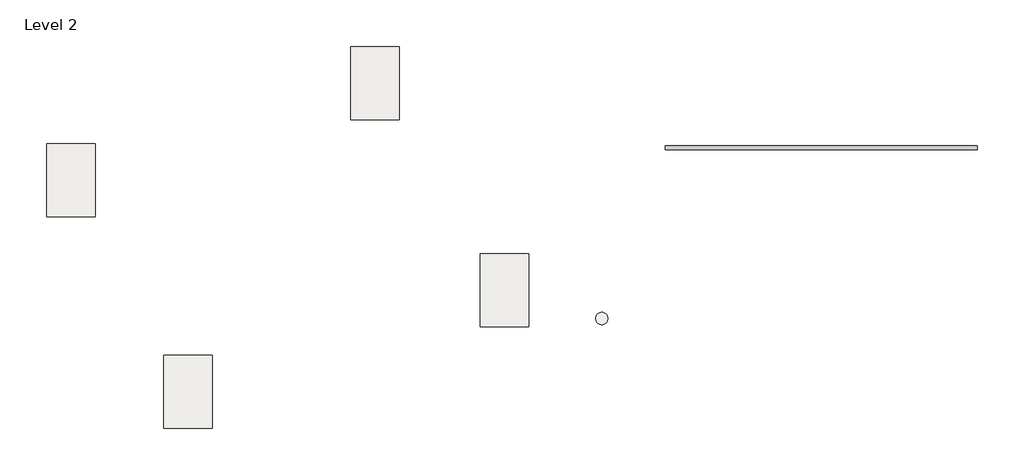
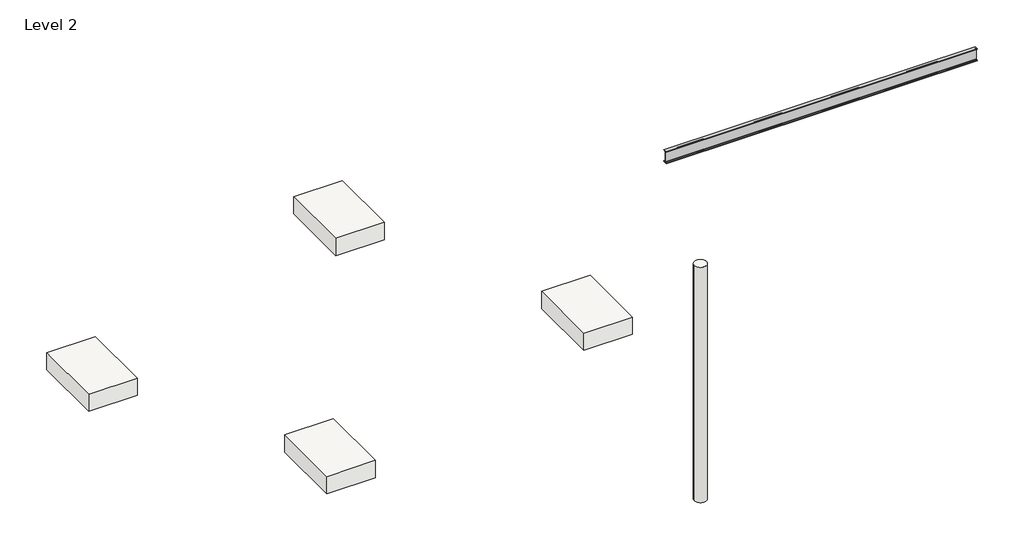
# One storey: 5 slabs, 1 beam.
"""IFC4 building model written with IfcOpenShell, lengths in millimetres."""

import ifcopenshell
import ifcopenshell.guid

model = None  # the IFC model being written
_history = None  # IfcOwnerHistory: only IFC2X3 demands one
_inside = {}  # id of a spatial element -> (the spatial element, [elements in it])
_under = {}  # id of a project, library or spatial element -> (it, [spatial elements below it])
_declared = {}  # id of a project -> (the project, [libraries it declares])
_typed = {}  # id of a type object -> (the type object, [elements of that type])
_made_of = {}  # id of a material, layer set ... -> (it, [elements and type objects made of it])


def new_model(schema):
    """Start an empty IFC model of exactly this schema.

    Asked for "IFC4X3", IfcOpenShell would pick the latest addendum, in which some entities
    have other attributes; the version numbers below select the first issue.
    IFC2X3 requires an IfcOwnerHistory on every rooted entity: one is made here for all.
    """
    global model, _history
    if schema == "IFC4X3":
        model = ifcopenshell.file(schema_version=(4, 3, 0, 0))
    else:
        model = ifcopenshell.file(schema=schema)
    _inside.clear()
    _under.clear()
    _declared.clear()
    _typed.clear()
    _made_of.clear()
    _history = None
    if model.schema == "IFC2X3":
        org = make("IfcOrganization", Name="unknown")
        user = make(
            "IfcPersonAndOrganization",
            ThePerson=make("IfcPerson", FamilyName="unknown"),
            TheOrganization=org,
        )
        app = make(
            "IfcApplication",
            ApplicationDeveloper=org,
            Version="unknown",
            ApplicationFullName="unknown",
            ApplicationIdentifier="unknown",
        )
        _history = make(
            "IfcOwnerHistory",
            OwningUser=user,
            OwningApplication=app,
            ChangeAction="ADDED",
            CreationDate=0,
        )
    return model


def make(cls, **values):
    """One entity of the class cls with the attributes given. An attribute that is None is left unset."""
    return model.create_entity(
        cls, **{name: value for name, value in values.items() if value is not None}
    )


def rooted(cls, **values):
    """An entity with a GlobalId (a new one), such as an element, a storey or a relation."""
    return make(cls, GlobalId=ifcopenshell.guid.new(), OwnerHistory=_history, **values)


def si_unit(unit_type, name, prefix=None):
    """IfcSIUnit, for example si_unit("LENGTHUNIT", "METRE", prefix="MILLI")."""
    return make("IfcSIUnit", UnitType=unit_type, Prefix=prefix, Name=name)


def assignment(units):
    """IfcUnitAssignment: the units of a project."""
    return None if units is None else make("IfcUnitAssignment", Units=units)


def point(xyz):
    """IfcCartesianPoint."""
    return None if xyz is None else make("IfcCartesianPoint", Coordinates=xyz)


def direction(xyz):
    """IfcDirection."""
    return None if xyz is None else make("IfcDirection", DirectionRatios=xyz)


def frame(location, z_axis=None, x_axis=None):
    """IfcAxis2Placement3D, a coordinate frame: its origin and axes. An axis left out is left unset."""
    return make(
        "IfcAxis2Placement3D",
        Location=point(location),
        Axis=direction(z_axis),
        RefDirection=direction(x_axis),
    )


def frame_2d(location, x_axis=None):
    """IfcAxis2Placement2D, a coordinate frame in the plane: its origin and x axis."""
    return make(
        "IfcAxis2Placement2D", Location=point(location), RefDirection=direction(x_axis)
    )


def origin():
    """The frame at (0, 0, 0) with its axes left unset."""
    return frame((0.0, 0.0, 0.0))


def origin_2d():
    """The frame at (0, 0) in the plane with its x axis left unset."""
    return frame_2d((0.0, 0.0))


def place(relative_to, where):
    """IfcLocalPlacement: puts the frame where relative to a parent placement (None: the world)."""
    return make(
        "IfcLocalPlacement", PlacementRelTo=relative_to, RelativePlacement=where
    )


def context(
    kind, dimensions, precision=None, world=None, true_north=None, identifier=None
):
    """IfcGeometricRepresentationContext, for example the 3D "Model" context."""
    return make(
        "IfcGeometricRepresentationContext",
        ContextIdentifier=identifier,
        ContextType=kind,
        CoordinateSpaceDimension=dimensions,
        Precision=precision,
        WorldCoordinateSystem=world,
        TrueNorth=true_north,
    )


def project(units=None, contexts=None):
    """IfcProject with its units and contexts."""
    return rooted(
        "IfcProject",
        Name="project",
        RepresentationContexts=contexts,
        UnitsInContext=assignment(units),
    )


def spatial(cls, under=None, at=None, **own):
    """A site, building, storey or space (cls), placed at a placement, below another one or the project."""
    s = rooted(cls, ObjectPlacement=at, **own)
    if under is not None:
        _under.setdefault(under.id(), (under, []))[1].append(s)
    return s


def polyline(points):
    """IfcPolyline through the points."""
    return make("IfcPolyline", Points=[point(p) for p in points])


def circle_curve(where, radius):
    """IfcCircle in the frame where."""
    return make("IfcCircle", Position=where, Radius=radius)


def trimmed(basis, trim1, trim2, sense, master):
    """IfcTrimmedCurve: the piece of a basis curve between two trims."""
    return make(
        "IfcTrimmedCurve",
        BasisCurve=basis,
        Trim1=trim1,
        Trim2=trim2,
        SenseAgreement=sense,
        MasterRepresentation=master,
    )


def segment(curve, same_sense, transition):
    """IfcCompositeCurveSegment."""
    return make(
        "IfcCompositeCurveSegment",
        Transition=transition,
        SameSense=same_sense,
        ParentCurve=curve,
    )


def composite_curve(segments, self_intersect=None):
    """IfcCompositeCurve: segments joined end to end."""
    return make("IfcCompositeCurve", Segments=segments, SelfIntersect=self_intersect)


def outline(outer, holes=None, kind="AREA"):
    """IfcArbitraryClosedProfileDef: a profile drawn as a closed curve; with holes, ...WithVoids."""
    if holes is None:
        return make("IfcArbitraryClosedProfileDef", ProfileType=kind, OuterCurve=outer)
    return make(
        "IfcArbitraryProfileDefWithVoids",
        ProfileType=kind,
        OuterCurve=outer,
        InnerCurves=holes,
    )


def extrude(swept, where, along, depth):
    """IfcExtrudedAreaSolid: the profile swept, set in the frame where, extruded along a direction by depth."""
    return make(
        "IfcExtrudedAreaSolid",
        SweptArea=swept,
        Position=where,
        ExtrudedDirection=direction(along),
        Depth=depth,
    )


def shape(context_of_items, identifier, shape_type, items):
    """IfcShapeRepresentation: the items that make up one representation, for example the "Body"."""
    return make(
        "IfcShapeRepresentation",
        ContextOfItems=context_of_items,
        RepresentationIdentifier=identifier,
        RepresentationType=shape_type,
        Items=items,
    )


def source(mapping_origin, context_of_items, identifier, shape_type, items):
    """IfcRepresentationMap: a shape defined once, which mapped items show again and again."""
    return make(
        "IfcRepresentationMap",
        MappingOrigin=mapping_origin,
        MappedRepresentation=shape(context_of_items, identifier, shape_type, items),
    )


def transform(
    local_origin,
    x_axis=None,
    y_axis=None,
    z_axis=None,
    scale=None,
    scale2=None,
    scale3=None,
    uniform=True,
):
    """IfcCartesianTransformationOperator3D, or its non-uniform kind. x_axis, y_axis, z_axis: its Axis1, 2, 3."""
    if uniform:
        return make(
            "IfcCartesianTransformationOperator3D",
            Axis1=direction(x_axis),
            Axis2=direction(y_axis),
            LocalOrigin=point(local_origin),
            Scale=scale,
            Axis3=direction(z_axis),
        )
    return make(
        "IfcCartesianTransformationOperator3DnonUniform",
        Axis1=direction(x_axis),
        Axis2=direction(y_axis),
        LocalOrigin=point(local_origin),
        Scale=scale,
        Axis3=direction(z_axis),
        Scale2=scale2,
        Scale3=scale3,
    )


def mapped(mapping_source, mapping_target):
    """IfcMappedItem: shows the shape of a source again, moved by a transform."""
    return make(
        "IfcMappedItem", MappingSource=mapping_source, MappingTarget=mapping_target
    )


def made_of(thing, what):
    """Note that an element or type object is made of a material, layer set ...; save() writes the relation."""
    if what is not None:
        _made_of.setdefault(what.id(), (what, []))[1].append(thing)
    return thing


def element(
    cls,
    number,
    at=None,
    inside=None,
    cuts=None,
    type_object=None,
    material=None,
    context=None,
    identifier="Body",
    shape_type=None,
    held_by="IfcProductDefinitionShape",
    body=None,
    shapes=None,
    **own,
):
    """One element of the class cls, such as IfcWall. Its Tag is "e" and its number.

    at: its placement. inside: the storey or other place that contains it. cuts: it is an
    opening in that element (IfcRelVoidsElement). A single representation is given by context,
    identifier, shape_type and body (its items); several are given by shapes. held_by: the class
    of the entity that holds the representations. save() writes the other relations.
    """
    e = rooted(cls, Tag="e%d" % number, ObjectPlacement=at, **own)
    if body is not None:
        shapes = [shape(context, identifier, shape_type, body)]
    if shapes is not None:
        e.Representation = make(held_by, Representations=shapes)
    if inside is not None:
        _inside.setdefault(inside.id(), (inside, []))[1].append(e)
    if cuts is not None:
        rooted(
            "IfcRelVoidsElement", RelatingBuildingElement=cuts, RelatedOpeningElement=e
        )
    if type_object is not None:
        _typed.setdefault(type_object.id(), (type_object, []))[1].append(e)
    return made_of(e, material)


def aggregate(whole, parts):
    """IfcRelAggregates: a whole, such as a stair, and the parts it consists of."""
    return rooted("IfcRelAggregates", RelatingObject=whole, RelatedObjects=parts)


def save(model, path):
    """Write the relations noted so far, then the file.

    IfcRelAggregates (storeys below a building ...), IfcRelContainedInSpatialStructure (elements
    in a storey), IfcRelDefinesByType, IfcRelAssociatesMaterial and IfcRelDeclares: one each for
    every whole, place, type object, material and project.
    """
    for whole, parts in _under.values():
        aggregate(whole, parts)
    for where, things in _inside.values():
        rooted(
            "IfcRelContainedInSpatialStructure",
            RelatedElements=things,
            RelatingStructure=where,
        )
    for kind, things in _typed.values():
        rooted("IfcRelDefinesByType", RelatedObjects=things, RelatingType=kind)
    for what, things in _made_of.values():
        rooted("IfcRelAssociatesMaterial", RelatedObjects=things, RelatingMaterial=what)
    for by, libraries in _declared.values():
        rooted("IfcRelDeclares", RelatingContext=by, RelatedDefinitions=libraries)
    model.write(path)


def ub_universal_beams_ub305x102x25_ce7b4b23(model_context):
    return source(origin(), model_context, "Body", "SweptSolid", [
        extrude(outline(composite_curve([segment(polyline([(50.8, -145.55), (50.8, -152.55), (-50.8, -152.55), (-50.8, -145.55), (-10.5, -145.55)]), True, "CONTINUOUS"), segment(trimmed(circle_curve(frame_2d((-10.5, -137.95)), 7.6), [point((-10.5, -145.55))], [point((-2.9, -137.95))], True, "CARTESIAN"), True, "CONTINUOUS"), segment(polyline([(-2.9, -137.95), (-2.9, 137.95)]), True, "CONTINUOUS"), segment(trimmed(circle_curve(frame_2d((-10.5, 137.95)), 7.6), [point((-2.9, 137.95))], [point((-10.5, 145.55))], True, "CARTESIAN"), True, "CONTINUOUS"), segment(polyline([(-10.5, 145.55), (-50.8, 145.55), (-50.8, 152.55), (50.8, 152.55), (50.8, 145.55), (10.5, 145.55)]), True, "CONTINUOUS"), segment(trimmed(circle_curve(frame_2d((10.5, 137.95)), 7.6), [point((10.5, 145.55))], [point((2.9, 137.95))], True, "CARTESIAN"), True, "CONTINUOUS"), segment(polyline([(2.9, 137.95), (2.9, -137.95)]), True, "CONTINUOUS"), segment(trimmed(circle_curve(frame_2d((10.5, -137.95)), 7.6), [point((2.9, -137.95))], [point((10.5, -145.55))], True, "CARTESIAN"), True, "CONTINUOUS"), segment(polyline([(10.5, -145.55), (50.8, -145.55)]), True, "CONTINUOUS")], self_intersect=False)), frame((-3850.0, 0.0, 0.0), z_axis=(1.0, 0.0, 0.0), x_axis=(0.0, 1.0, 0.0)), (0.0, 0.0, 1.0), 7700.0),
    ])


def footing_rectangular_1800_x_1200_x_450mm_16ba7ea5(model_context):
    return source(origin(), model_context, "Body", "SweptSolid", [
        extrude(outline(polyline([(600.0, 900.0), (600.0, -900.0), (-600.0, -900.0), (-600.0, 900.0), (600.0, 900.0)])), frame((0.0, 0.0, -450.0), z_axis=(0.0, 0.0, 1.0), x_axis=(1.0, 0.0, 0.0)), (0.0, 0.0, 1.0), 450.0),
    ])


def m_pile_steel_pipe_300mm_diameter_9db3f09c(model_context):
    return source(origin(), model_context, "Body", "SweptSolid", [
        extrude(outline(composite_curve([segment(trimmed(circle_curve(origin_2d(), 150.0), [point((-150.0, 0.0))], [point((150.0, 0.0))], False, "CARTESIAN"), True, "CONTINUOUS"), segment(trimmed(circle_curve(origin_2d(), 150.0), [point((150.0, 0.0))], [point((-150.0, 0.0))], False, "CARTESIAN"), True, "CONTINUOUS")], self_intersect=False)), frame((0.0, 0.0, -6000.0), z_axis=(0.0, 0.0, 1.0), x_axis=(1.0, 0.0, 0.0)), (0.0, 0.0, 1.0), 6150.0),
    ])


model = new_model("IFC4")

# Units and contexts
model_context = context("Model", 3, world=origin())
ifc_project = project(units=[si_unit("LENGTHUNIT", "METRE", prefix="MILLI")], contexts=[model_context])

# Site, building, storey
site = spatial("IfcSite", under=ifc_project)
building = spatial("IfcBuilding", under=site)
storey = spatial("IfcBuildingStorey", under=building, Name="Level 2", Elevation=3000.0)

# Beam
placement = place(None, origin())
ub_universal_beams_ub305x102x25_shape = ub_universal_beams_ub305x102x25_ce7b4b23(model_context)
element("IfcBeam", 1, ObjectType="UB-Universal Beams : UB305x102x25", at=placement, inside=storey, context=model_context, shape_type="MappedRepresentation", body=[
    mapped(ub_universal_beams_ub305x102x25_shape, transform((28868.6903069, 5320.2701011, 2847.45), x_axis=(1.0, 0.0, 0.0), y_axis=(0.0, 1.0, 0.0), z_axis=(0.0, 0.0, 1.0))),
])

# Slabs
footing_rectangular_1800_x_1200_x_450mm_shape = footing_rectangular_1800_x_1200_x_450mm_16ba7ea5(model_context)
element("IfcSlab", 2, ObjectType="Footing-Rectangular : 1800 x 1200 x 450mm", at=placement, inside=storey, context=model_context, shape_type="MappedRepresentation", body=[
    mapped(footing_rectangular_1800_x_1200_x_450mm_shape, transform((10369.0414459, 4518.4031293, 3000.0), x_axis=(1.0, 0.0, 0.0), y_axis=(0.0, 1.0, 0.0), z_axis=(0.0, 0.0, 1.0))),
])
element("IfcSlab", 3, ObjectType="Footing-Rectangular : 1800 x 1200 x 450mm", at=placement, inside=storey, context=model_context, shape_type="MappedRepresentation", body=[
    mapped(footing_rectangular_1800_x_1200_x_450mm_shape, transform((17864.2414459, 6913.6031293, 3000.0), x_axis=(1.0, 0.0, 0.0), y_axis=(0.0, 1.0, 0.0), z_axis=(0.0, 0.0, 1.0))),
])
element("IfcSlab", 4, ObjectType="Footing-Rectangular : 1800 x 1200 x 450mm", at=placement, inside=storey, context=model_context, shape_type="MappedRepresentation", body=[
    mapped(footing_rectangular_1800_x_1200_x_450mm_shape, transform((21059.4414459, 1808.8031293, 2500.0), x_axis=(1.0, 0.0, 0.0), y_axis=(0.0, 1.0, 0.0), z_axis=(0.0, 0.0, 1.0))),
])
element("IfcSlab", 5, ObjectType="Footing-Rectangular : 1800 x 1200 x 450mm", at=placement, inside=storey, context=model_context, shape_type="MappedRepresentation", body=[
    mapped(footing_rectangular_1800_x_1200_x_450mm_shape, transform((13254.6414459, -695.9968707, 3000.0), x_axis=(1.0, 0.0, 0.0), y_axis=(0.0, 1.0, 0.0), z_axis=(0.0, 0.0, 1.0))),
])
m_pile_steel_pipe_300mm_diameter_shape = m_pile_steel_pipe_300mm_diameter_9db3f09c(model_context)
element("IfcSlab", 6, ObjectType="M_Pile-Steel Pipe : 300mm Diameter", at=placement, inside=storey, context=model_context, shape_type="MappedRepresentation", body=[
    mapped(m_pile_steel_pipe_300mm_diameter_shape, transform((23459.4414459, 1108.8031293, 3000.0), x_axis=(1.0, 0.0, 0.0), y_axis=(0.0, 1.0, 0.0), z_axis=(0.0, 0.0, 1.0))),
])

save(model, "model.ifc")

# Revit data of these elements
# Project information
#   Project Issue Date = "Issue Date"
#   Project Status = "Project Status"
#   Client Name = "Owner"
#   Project Address = "Enter address here"
#   Project Name = "Project Name"
#   Project Number = "Project Number"
# Type "UB-Universal Beams : UB305x102x25"
#   Section Name Key = "UB305X102X25"
#   Width = 10.16 cm
#   Web Thickness = 0.58 cm
#   Web Fillet = 0.76 cm
#   Warping Constant = 27300.0 cm⁶
#   Torsional Moment of Inertia = 4.77 cm⁴
#   Section Area = 31.6 cm²
#   Plastic Modulus weak axis = 39.0 cm³
#   Plastic Modulus strong axis = 342.0 cm³
#   Nominal Weight = 24.7999 kgf/m
#   Moment of Inertia weak axis = 123.00 cm⁴
#   Moment of Inertia strong axis = 4455.00 cm⁴
#   Height = 30.51 cm
#   Flange Thickness = 0.7 cm
#   Elastic Modulus weak axis = 24.2 cm³
#   Elastic Modulus strong axis = 292.0 cm³
#   Centroid Vertical = 15.255 cm
#   Centroid Horizontal = 5.08 cm
#   Bolt Spacing = 5.4 cm
#   Length [instance default] = 1500 mm
#   Structural Material [instance default] = Metal - Steel 43-275
#   Type Comments = ""
#   Assembly Code = ""
# Type "Footing-Rectangular : 1800 x 1200 x 450mm"
#   Width = 1200 mm
#   Length = 1800 mm
#   Foundation Thickness = 450 mm
#   Structural Material [instance default] = Concrete - Cast-in-Place Concrete
#   Assembly Code = ""
# Type "M_Pile-Steel Pipe : 300mm Diameter"
#   Assembly Code = "A1020130"
#   Radius = 150 mm
#   Minimum Embedment = 150 mm
#   Diameter = 300 mm
#   Depth = 6000 mm
#   Structural Material [instance default] = Steel, 45-345
# Element 1 (IfcBeam, "UB-Universal Beams : UB305x102x25")
#   Structural Material = Metal - Steel 43-275
#   Phase Created = New Construction
#   Materials on its faces: "Metal - Steel 43-275"
# Element 2 (IfcSlab, "Footing-Rectangular : 1800 x 1200 x 450mm")
#   Easting = "10.587"
#   Cut Off = "2.918"
#   Northing = "2.317"
#   Dbl_X = 0
#   Dbl_Y = 0
#   Dbl_Z = 0
#   Structural Material = Concrete - Cast-in-Place Concrete
#   Phase Created = New Construction
#   Materials on its faces: "Concrete - Cast-in-Place Concrete"
# Element 3 (IfcSlab, "Footing-Rectangular : 1800 x 1200 x 450mm")
#   Easting = "18.449"
#   Cut Off = "2.918"
#   Northing = "2.004"
#   Dbl_X = 0
#   Dbl_Y = 0
#   Dbl_Z = 0
#   Structural Material = Concrete - Cast-in-Place Concrete
#   Phase Created = New Construction
#   Materials on its faces: "Concrete - Cast-in-Place Concrete"
# Element 4 (IfcSlab, "Footing-Rectangular : 1800 x 1200 x 450mm")
#   Easting = "19.706"
#   Cut Off = "2.418"
#   Northing = "-3.885"
#   Dbl_X = 0
#   Dbl_Y = 0
#   Dbl_Z = 0
#   Structural Material = Concrete - Cast-in-Place Concrete
#   Phase Created = New Construction
#   Materials on its faces: "Concrete - Cast-in-Place Concrete"
# Element 5 (IfcSlab, "Footing-Rectangular : 1800 x 1200 x 450mm")
#   Easting = "11.515"
#   Cut Off = "2.918"
#   Northing = "-3.570"
#   Dbl_X = 0
#   Dbl_Y = 0
#   Dbl_Z = 0
#   Structural Material = Concrete - Cast-in-Place Concrete
#   Phase Created = New Construction
#   Materials on its faces: "Concrete - Cast-in-Place Concrete"
# Element 6 (IfcSlab, "M_Pile-Steel Pipe : 300mm Diameter")
#   Structural Material = Steel, 45-345
#   Phase Created = New Construction
#   Materials on its faces: "Steel, 45-345"
# Materials
#   "Metal - Steel 43-275": class "Metal", colour RGB 247 247 247, transparency 0, Cost = 0
#   "Concrete - Cast-in-Place Concrete": class "Concrete", colour RGB 192 192 192, transparency 0, Cost = 0
#   "Steel, 45-345": class "Metal", colour RGB 247 247 247, transparency 0, Description = "Steel 345 MPa", Cost = 0
